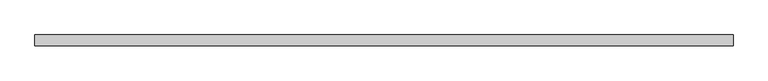
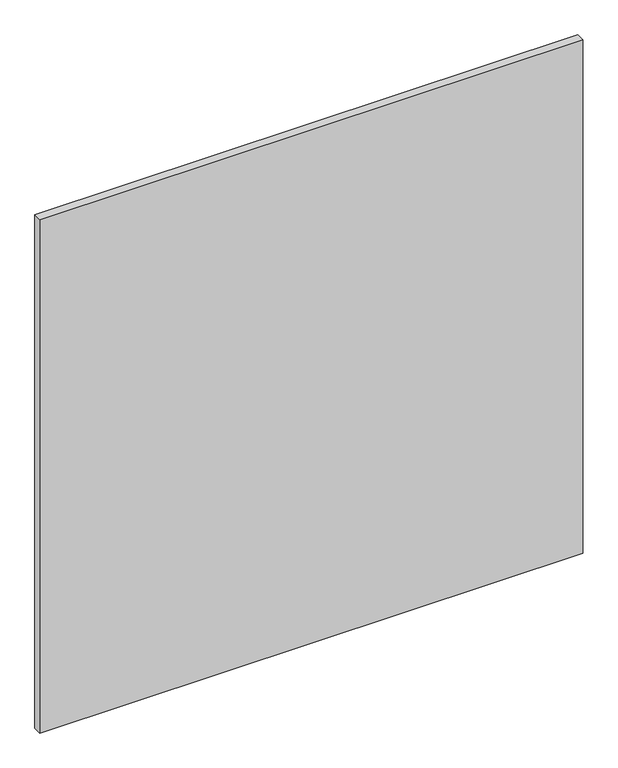
"""IFC4 building model written with IfcOpenShell, lengths in millimetres: proxy geometry, Inner panel:Inner panel:1:Inner panel:1 : Inner panel:Inner panel:300324:300043:Inner panel:1:Inner panel:1 : Inner panel:Inner panel:300324:300043 : Inner panel:Inner panel:1:Inner panel:1 : Inner panel:Inner panel:300324:300043:36 : Inner panel:Inner panel:1:Inner panel:1 : Inner panel:Inner panel:300324:300043:Inner panel:1:Inner panel:1 : Inner panel:Inner panel:300324:300043 : Inner panel:Inner panel:1:Inner panel:1 : Inner panel:Inner panel:300324:300043:300031."""

from ifc_helpers import new_model, si_unit, frame, origin, place, context, project, spatial, polyline, outline, extrude, source, transform, mapped, element, save


def generic_models_4b9c950b(model_context):
    return source(origin(), model_context, "Body", "SweptSolid", [
        extrude(outline(polyline([(594963.6367239, -578778.4413841), (596182.8367239, -578778.4413841), (596182.8367239, -578797.4913841), (594963.6367239, -578797.4913841), (594963.6367239, -578778.4413841)])), frame((0.0, 0.0, 1270.0), z_axis=(0.0, 0.0, 1.0), x_axis=(1.0, 0.0, 0.0)), (0.0, 0.0, 1.0), 1219.2),
    ])


if __name__ == "__main__":
    model = new_model("IFC4")
    model_context = context("Model", 3, world=origin())
    ifc_project = project(units=[si_unit("LENGTHUNIT", "METRE", prefix="MILLI")], contexts=[model_context])
    site = spatial("IfcSite", under=ifc_project)
    building = spatial("IfcBuilding", under=site)
    placement = place(None, origin())
    generic_models_shape = generic_models_4b9c950b(model_context)
    element("IfcBuildingElementProxy", 1, Name="Inner panel:Inner panel:1:Inner panel:1 : Inner panel:Inner panel:300324:300043:Inner panel:1:Inner panel:1 : Inner panel:Inner panel:300324:300043 : Inner panel:Inner panel:1:Inner panel:1 : Inner panel:Inner panel:300324:300043:36 : Inner panel:Inner panel:1:Inner panel:1 : Inner panel:Inner panel:300324:300043:Inner panel:1:Inner panel:1 : Inner panel:Inner panel:300324:300043 : Inner panel:Inner panel:1:Inner panel:1 : Inner panel:Inner panel:300324:300043:300031", ObjectType="Inner panel:Inner panel:1:Inner panel:1 : Inner panel:Inner panel:300324:300043:Inner panel:1:Inner panel:1 : Inner panel:Inner panel:300324:300043 : Inner panel:Inner panel:1:Inner panel:1 : Inner panel:Inner panel:300324:300043:36 : Inner panel:Inner panel:1:Inner panel:1 : Inner panel:Inner panel:300324:300043:Inner panel:1:Inner panel:1 : Inner panel:Inner panel:300324:300043 : Inner panel:Inner panel:1:Inner panel:1 : Inner panel:Inner panel:300324:300043:300031", at=placement, inside=building, context=model_context, shape_type="MappedRepresentation", body=[
        mapped(generic_models_shape, transform((0.0, 0.0, 0.0), x_axis=(1.0, 0.0, 0.0), y_axis=(0.0, 1.0, 0.0), z_axis=(0.0, 0.0, 1.0))),
    ])
    save(model, "model.ifc")

# Revit data of these elements
# Type "Inner panel:Inner panel:1:Inner panel:1 : Inner panel:Inner panel:300324:300043:Inner panel:1:Inner panel:1 : Inner panel:Inner panel:300324:300043 : Inner panel:Inner panel:1:Inner panel:1 : Inner panel:Inner panel:300324:300043:36 : Inner panel:Inner panel:1:Inner panel:1 : Inner panel:Inner panel:300324:300043:Inner panel:1:Inner panel:1 : Inner panel:Inner panel:300324:300043 : Inner panel:Inner panel:1:Inner panel:1 : Inner panel:Inner panel:300324:300043:300031"
#   NameOverride = "Inner panel:Inner panel:1:Inner panel:1 : Inner panel:Inner panel:300324:300043:Inner panel:1:Inner panel:1 : Inner panel:Inner panel:300324:300043 : Inner panel:Inner panel:1:Inner panel:1 : Inner panel:Inner panel:300324:300043:300031"
#   ObjectTypeOverride = "Inner panel:1:Inner panel:1 : Inner panel:Inner panel:300324:300043 : Inner panel:Inner panel:1:Inner panel:1 : Inner panel:Inner panel:300324:300043"
#   Reference = "Inner panel"
#   Tag = "300031"
# Element 1 (IfcBuildingElementProxy, "Inner panel:Inner panel:1:Inner panel:1 : Inner panel:Inner panel:300324:300043:Inner panel:1:Inner panel:1 : Inner panel:Inner panel:300324:300043 : Inner panel:Inner panel:1:Inner panel:1 : Inner panel:Inner panel:300324:300043:36 : Inner panel:Inner panel:1:Inner panel:1 : Inner panel:Inner panel:300324:300043:Inner panel:1:Inner panel:1 : Inner panel:Inner panel:300324:300043 : Inner panel:Inner panel:1:Inner panel:1 : Inner panel:Inner panel:300324:300043:300031")
#   Materials on its faces: "¾” (CLASS A) FIRE RETARDANT PLYWOOD ...OR… IF 1/4\" GYP. BD UNDER PLYWOOD, FLAME SPREAD TO BE CLASS C -  (FINISH: GRADE B - PREFINISHED STAINED/SEALED) - 1/4\" GAP BTWN PANELS (FASTENERS T.B.D.)"
# Materials
#   "¾” (CLASS A) FIRE RETARDANT PLYWOOD ...OR… IF 1/4\" GYP. BD UNDER PLYWOOD, FLAME SPREAD TO BE CLASS C -  (FINISH: GRADE B - PREFINISHED STAINED/SEALED) - 1/4\" GAP BTWN PANELS (FASTENERS T.B.D.)": class "Wood", colour RGB 149 120 74, transparency 0, Description = "Plywood, sheathing grade", Cost = 0
